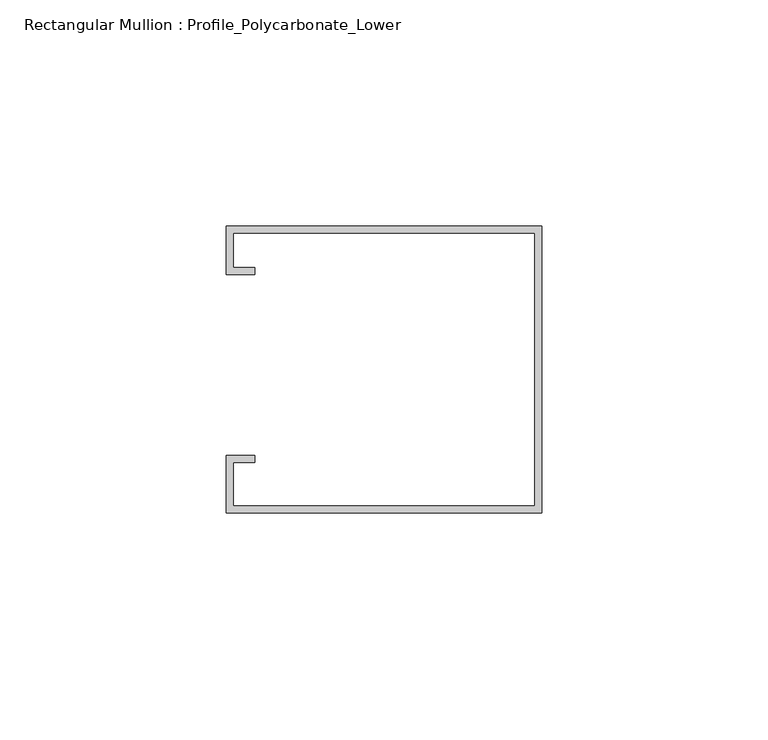
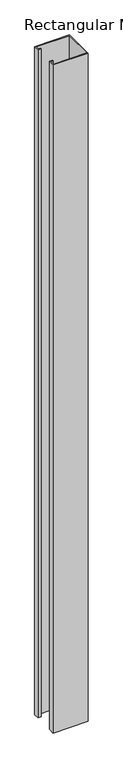
"""IFC4 building model written with IfcOpenShell, lengths in millimetres: member geometry, Rectangular Mullion : Profile_Polycarbonate_Lower."""

import ifcopenshell
import ifcopenshell.guid

model = None  # the IFC model being written
_history = None  # IfcOwnerHistory: only IFC2X3 demands one
_inside = {}  # id of a spatial element -> (the spatial element, [elements in it])
_under = {}  # id of a project, library or spatial element -> (it, [spatial elements below it])
_declared = {}  # id of a project -> (the project, [libraries it declares])
_typed = {}  # id of a type object -> (the type object, [elements of that type])
_made_of = {}  # id of a material, layer set ... -> (it, [elements and type objects made of it])


def new_model(schema):
    """Start an empty IFC model of exactly this schema.

    Asked for "IFC4X3", IfcOpenShell would pick the latest addendum, in which some entities
    have other attributes; the version numbers below select the first issue.
    IFC2X3 requires an IfcOwnerHistory on every rooted entity: one is made here for all.
    """
    global model, _history
    if schema == "IFC4X3":
        model = ifcopenshell.file(schema_version=(4, 3, 0, 0))
    else:
        model = ifcopenshell.file(schema=schema)
    _inside.clear()
    _under.clear()
    _declared.clear()
    _typed.clear()
    _made_of.clear()
    _history = None
    if model.schema == "IFC2X3":
        org = make("IfcOrganization", Name="unknown")
        user = make(
            "IfcPersonAndOrganization",
            ThePerson=make("IfcPerson", FamilyName="unknown"),
            TheOrganization=org,
        )
        app = make(
            "IfcApplication",
            ApplicationDeveloper=org,
            Version="unknown",
            ApplicationFullName="unknown",
            ApplicationIdentifier="unknown",
        )
        _history = make(
            "IfcOwnerHistory",
            OwningUser=user,
            OwningApplication=app,
            ChangeAction="ADDED",
            CreationDate=0,
        )
    return model


def make(cls, **values):
    """One entity of the class cls with the attributes given. An attribute that is None is left unset."""
    return model.create_entity(
        cls, **{name: value for name, value in values.items() if value is not None}
    )


def rooted(cls, **values):
    """An entity with a GlobalId (a new one), such as an element, a storey or a relation."""
    return make(cls, GlobalId=ifcopenshell.guid.new(), OwnerHistory=_history, **values)


def si_unit(unit_type, name, prefix=None):
    """IfcSIUnit, for example si_unit("LENGTHUNIT", "METRE", prefix="MILLI")."""
    return make("IfcSIUnit", UnitType=unit_type, Prefix=prefix, Name=name)


def assignment(units):
    """IfcUnitAssignment: the units of a project."""
    return None if units is None else make("IfcUnitAssignment", Units=units)


def point(xyz):
    """IfcCartesianPoint."""
    return None if xyz is None else make("IfcCartesianPoint", Coordinates=xyz)


def direction(xyz):
    """IfcDirection."""
    return None if xyz is None else make("IfcDirection", DirectionRatios=xyz)


def frame(location, z_axis=None, x_axis=None):
    """IfcAxis2Placement3D, a coordinate frame: its origin and axes. An axis left out is left unset."""
    return make(
        "IfcAxis2Placement3D",
        Location=point(location),
        Axis=direction(z_axis),
        RefDirection=direction(x_axis),
    )


def origin():
    """The frame at (0, 0, 0) with its axes left unset."""
    return frame((0.0, 0.0, 0.0))


def place(relative_to, where):
    """IfcLocalPlacement: puts the frame where relative to a parent placement (None: the world)."""
    return make(
        "IfcLocalPlacement", PlacementRelTo=relative_to, RelativePlacement=where
    )


def context(
    kind, dimensions, precision=None, world=None, true_north=None, identifier=None
):
    """IfcGeometricRepresentationContext, for example the 3D "Model" context."""
    return make(
        "IfcGeometricRepresentationContext",
        ContextIdentifier=identifier,
        ContextType=kind,
        CoordinateSpaceDimension=dimensions,
        Precision=precision,
        WorldCoordinateSystem=world,
        TrueNorth=true_north,
    )


def project(units=None, contexts=None):
    """IfcProject with its units and contexts."""
    return rooted(
        "IfcProject",
        Name="project",
        RepresentationContexts=contexts,
        UnitsInContext=assignment(units),
    )


def spatial(cls, under=None, at=None, **own):
    """A site, building, storey or space (cls), placed at a placement, below another one or the project."""
    s = rooted(cls, ObjectPlacement=at, **own)
    if under is not None:
        _under.setdefault(under.id(), (under, []))[1].append(s)
    return s


def polyline(points):
    """IfcPolyline through the points."""
    return make("IfcPolyline", Points=[point(p) for p in points])


def outline(outer, holes=None, kind="AREA"):
    """IfcArbitraryClosedProfileDef: a profile drawn as a closed curve; with holes, ...WithVoids."""
    if holes is None:
        return make("IfcArbitraryClosedProfileDef", ProfileType=kind, OuterCurve=outer)
    return make(
        "IfcArbitraryProfileDefWithVoids",
        ProfileType=kind,
        OuterCurve=outer,
        InnerCurves=holes,
    )


def extrude(swept, where, along, depth):
    """IfcExtrudedAreaSolid: the profile swept, set in the frame where, extruded along a direction by depth."""
    return make(
        "IfcExtrudedAreaSolid",
        SweptArea=swept,
        Position=where,
        ExtrudedDirection=direction(along),
        Depth=depth,
    )


def shape(context_of_items, identifier, shape_type, items):
    """IfcShapeRepresentation: the items that make up one representation, for example the "Body"."""
    return make(
        "IfcShapeRepresentation",
        ContextOfItems=context_of_items,
        RepresentationIdentifier=identifier,
        RepresentationType=shape_type,
        Items=items,
    )


def source(mapping_origin, context_of_items, identifier, shape_type, items):
    """IfcRepresentationMap: a shape defined once, which mapped items show again and again."""
    return make(
        "IfcRepresentationMap",
        MappingOrigin=mapping_origin,
        MappedRepresentation=shape(context_of_items, identifier, shape_type, items),
    )


def transform(
    local_origin,
    x_axis=None,
    y_axis=None,
    z_axis=None,
    scale=None,
    scale2=None,
    scale3=None,
    uniform=True,
):
    """IfcCartesianTransformationOperator3D, or its non-uniform kind. x_axis, y_axis, z_axis: its Axis1, 2, 3."""
    if uniform:
        return make(
            "IfcCartesianTransformationOperator3D",
            Axis1=direction(x_axis),
            Axis2=direction(y_axis),
            LocalOrigin=point(local_origin),
            Scale=scale,
            Axis3=direction(z_axis),
        )
    return make(
        "IfcCartesianTransformationOperator3DnonUniform",
        Axis1=direction(x_axis),
        Axis2=direction(y_axis),
        LocalOrigin=point(local_origin),
        Scale=scale,
        Axis3=direction(z_axis),
        Scale2=scale2,
        Scale3=scale3,
    )


def mapped(mapping_source, mapping_target):
    """IfcMappedItem: shows the shape of a source again, moved by a transform."""
    return make(
        "IfcMappedItem", MappingSource=mapping_source, MappingTarget=mapping_target
    )


def made_of(thing, what):
    """Note that an element or type object is made of a material, layer set ...; save() writes the relation."""
    if what is not None:
        _made_of.setdefault(what.id(), (what, []))[1].append(thing)
    return thing


def element(
    cls,
    number,
    at=None,
    inside=None,
    cuts=None,
    type_object=None,
    material=None,
    context=None,
    identifier="Body",
    shape_type=None,
    held_by="IfcProductDefinitionShape",
    body=None,
    shapes=None,
    **own,
):
    """One element of the class cls, such as IfcWall. Its Tag is "e" and its number.

    at: its placement. inside: the storey or other place that contains it. cuts: it is an
    opening in that element (IfcRelVoidsElement). A single representation is given by context,
    identifier, shape_type and body (its items); several are given by shapes. held_by: the class
    of the entity that holds the representations. save() writes the other relations.
    """
    e = rooted(cls, Tag="e%d" % number, ObjectPlacement=at, **own)
    if body is not None:
        shapes = [shape(context, identifier, shape_type, body)]
    if shapes is not None:
        e.Representation = make(held_by, Representations=shapes)
    if inside is not None:
        _inside.setdefault(inside.id(), (inside, []))[1].append(e)
    if cuts is not None:
        rooted(
            "IfcRelVoidsElement", RelatingBuildingElement=cuts, RelatedOpeningElement=e
        )
    if type_object is not None:
        _typed.setdefault(type_object.id(), (type_object, []))[1].append(e)
    return made_of(e, material)


def aggregate(whole, parts):
    """IfcRelAggregates: a whole, such as a stair, and the parts it consists of."""
    return rooted("IfcRelAggregates", RelatingObject=whole, RelatedObjects=parts)


def save(model, path):
    """Write the relations noted so far, then the file.

    IfcRelAggregates (storeys below a building ...), IfcRelContainedInSpatialStructure (elements
    in a storey), IfcRelDefinesByType, IfcRelAssociatesMaterial and IfcRelDeclares: one each for
    every whole, place, type object, material and project.
    """
    for whole, parts in _under.values():
        aggregate(whole, parts)
    for where, things in _inside.values():
        rooted(
            "IfcRelContainedInSpatialStructure",
            RelatedElements=things,
            RelatingStructure=where,
        )
    for kind, things in _typed.values():
        rooted("IfcRelDefinesByType", RelatedObjects=things, RelatingType=kind)
    for what, things in _made_of.values():
        rooted("IfcRelAssociatesMaterial", RelatedObjects=things, RelatingMaterial=what)
    for by, libraries in _declared.values():
        rooted("IfcRelDeclares", RelatingContext=by, RelatedDefinitions=libraries)
    model.write(path)


def rectangular_mullion_profile_polycarbonate_lower_301292b8(model_context):
    return source(origin(), model_context, "Body", "SweptSolid", [
        extrude(outline(polyline([(0.0, -32.7), (-69.85, -32.7), (-69.85, -20.0), (-63.5, -20.0), (-63.5, -21.5875), (-68.2625, -21.5875), (-68.2625, -31.1125), (-1.5875, -31.1125), (-1.5875, 29.2125), (-68.2625, 29.2125), (-68.2625, 21.5875), (-63.5, 21.5875), (-63.5, 20.0), (-69.85, 20.0), (-69.85, 30.8), (0.0, 30.8), (0.0, -32.7)])), frame((0.0, 0.0, -1409.7), z_axis=(0.0, 0.0, 1.0), x_axis=(1.0, 0.0, 0.0)), (0.0, 0.0, 1.0), 1409.7),
    ])


if __name__ == "__main__":
    model = new_model("IFC4")
    model_context = context("Model", 3, world=origin())
    ifc_project = project(units=[si_unit("LENGTHUNIT", "METRE", prefix="MILLI")], contexts=[model_context])
    site = spatial("IfcSite", under=ifc_project)
    building = spatial("IfcBuilding", under=site)
    placement = place(None, origin())
    rectangular_mullion_profile_polycarbonate_lower_shape = rectangular_mullion_profile_polycarbonate_lower_301292b8(model_context)
    element("IfcMember", 1, ObjectType="Rectangular Mullion : Profile_Polycarbonate_Lower", at=placement, inside=building, context=model_context, shape_type="MappedRepresentation", body=[
        mapped(rectangular_mullion_profile_polycarbonate_lower_shape, transform((0.0, 0.0, 0.0), x_axis=(1.0, 0.0, 0.0), y_axis=(0.0, 1.0, 0.0), z_axis=(0.0, 0.0, 1.0))),
    ])
    save(model, "model.ifc")

# Revit data of these elements
# Type "Rectangular Mullion : Profile_Polycarbonate_Lower"
#   built-in parameter 1007322 = 0.208333 (stored number, unit not read)
#   built-in parameter 1007321 = 0 (stored number, unit not read)
#   built-in parameter 1007320 = 0.00520833 (stored number, unit not read)
# Element 1 (IfcMember, "Rectangular Mullion : Profile_Polycarbonate_Lower")
#   Materials on its faces: "ALUMINUM PROFILE AT POLYCARBONATE PANEL"
# Materials
#   "ALUMINUM PROFILE AT POLYCARBONATE PANEL": class "Metal", colour RGB 244 244 244, transparency 0, Description = "Aluminum 6061", Cost = 0
